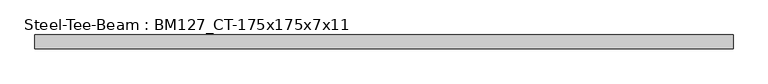
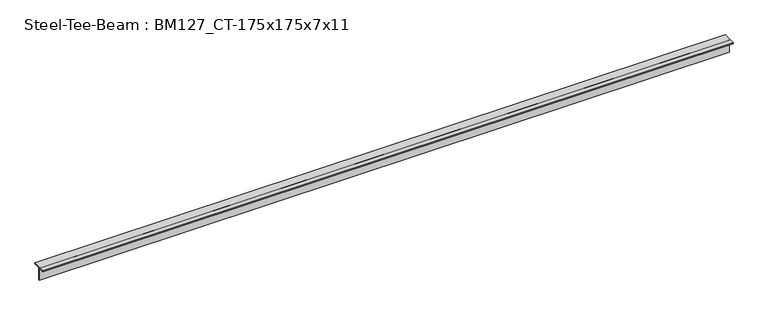
"""IFC4 building model written with IfcOpenShell, lengths in millimetres: beam geometry, Steel-Tee-Beam : BM127_CT-175x175x7x11."""

from ifc_helpers import new_model, si_unit, point, frame, frame_2d, origin, place, context, project, spatial, polyline, circle_curve, trimmed, segment, composite_curve, outline, extrude, source, transform, mapped, element, save


def steel_tee_beam_bm127_ct_175x175x7x11_3d5bc00e(model_context):
    return source(origin(), model_context, "Body", "SweptSolid", [
        extrude(outline(composite_curve([segment(polyline([(87.5, 87.5), (87.5, 76.5), (17.5, 76.5)]), True, "CONTINUOUS"), segment(trimmed(circle_curve(frame_2d((17.5, 62.5)), 14.0), [point((17.5, 76.5))], [point((3.5, 62.5))], True, "CARTESIAN"), True, "CONTINUOUS"), segment(polyline([(3.5, 62.5), (3.5, -87.5), (-3.5, -87.5), (-3.5, 62.5)]), True, "CONTINUOUS"), segment(trimmed(circle_curve(frame_2d((-17.5, 62.5)), 14.0), [point((-3.5, 62.5))], [point((-17.5, 76.5))], True, "CARTESIAN"), True, "CONTINUOUS"), segment(polyline([(-17.5, 76.5), (-87.5, 76.5), (-87.5, 87.5), (87.5, 87.5)]), True, "CONTINUOUS")], self_intersect=False)), frame((-4298.1792655, 0.0, 0.0), z_axis=(1.0, 0.0, 0.0), x_axis=(0.0, 1.0, 0.0)), (0.0, 0.0, 1.0), 8725.555017),
    ])


if __name__ == "__main__":
    model = new_model("IFC4")
    model_context = context("Model", 3, world=origin())
    ifc_project = project(units=[si_unit("LENGTHUNIT", "METRE", prefix="MILLI")], contexts=[model_context])
    site = spatial("IfcSite", under=ifc_project)
    building = spatial("IfcBuilding", under=site)
    placement = place(None, origin())
    steel_tee_beam_bm127_ct_175x175x7x11_shape = steel_tee_beam_bm127_ct_175x175x7x11_3d5bc00e(model_context)
    element("IfcBeam", 1, ObjectType="Steel-Tee-Beam : BM127_CT-175x175x7x11", at=placement, inside=building, context=model_context, shape_type="MappedRepresentation", body=[
        mapped(steel_tee_beam_bm127_ct_175x175x7x11_shape, transform((0.0, 0.0, 0.0), x_axis=(1.0, 0.0, 0.0), y_axis=(0.0, 1.0, 0.0), z_axis=(0.0, 0.0, 1.0))),
    ])
    save(model, "model.ifc")

# Revit data of these elements
# Type "Steel-Tee-Beam : BM127_CT-175x175x7x11"
#   Section Area = 31.57 cm²
#   Mass per Unit Length = 24.80 kg/m
#   Length [instance default] = 1524 mm
#   bf = 175 mm
#   d = 175 mm
#   k = 25 mm
#   kr = 14 mm
#   tf = 11 mm
#   tw = 7 mm
#   hec_material4 [instance default] = none
#   hec_material3 [instance default] = none
#   hec_material2 [instance default] = none
#   hec_material1 [instance default] = none
#   Structural Material [instance default] = Steel, 45-345
#   Assembly Code = ""
# Element 1 (IfcBeam, "Steel-Tee-Beam : BM127_CT-175x175x7x11")
#   hec_material3 = F01AC000-00002_Building/Shelter Fire Proofing Work_Intumescent Coating Type_1 hr. rating (UL 1709))
#   hec_material1 = S03AA029-00001_Main Steel Structure Erection Work_Shelter/Building_Light Steel
#   Structural Material = S01AA003-00001_Main Steel Structure Fabrication Work_Shelter/Building_Light Steel - Standard
#   Materials on its faces: "S01AA003-00001_Main Steel Structure Fabrication Work_Shelter/Building_Light Steel - Standard"
# Materials
#   "Steel, 45-345": class "Metal", colour RGB 189 187 185, transparency 0, Description = "Steel 345 MPa", Cost = 0
#   "S01AA003-00001_Main Steel Structure Fabrication Work_Shelter/Building_Light Steel - Standard": class "Metal", colour RGB 120 120 120, transparency 0, Comments = "(30KG/M>Weight)", Description = "Structural steel 50ksi", W00) Work Master Code = "S01AA003-00001", W01) Work Master_Lv1 = "Main Steel Structure Fabrication Work", W02) Work Master_Lv2 = "Shelter/Building", W03) Work Master_Spec.1 = "Light Steel - Standard (30KG/M>Weight)", Cost = 0
#   "F01AC000-00002_Building/Shelter Fire Proofing Work_Intumescent Coating Type_1 hr. rating (UL 1709))": class "Metal", colour RGB 255 128 128, transparency 0, Description = "Paint finished steel", W00) Work Master Code = "F01AC000-00002", W01) Work Master_Lv1 = "Building/Shelter Fire Proofing Work", W02) Work Master_Lv2 = "Intumescent Coating Type", W03) Work Master_Spec.1 = "1 hr. rating (UL 1709)", Cost = 0
#   "S03AA029-00001_Main Steel Structure Erection Work_Shelter/Building_Light Steel": class "Metal", colour RGB 120 120 120, transparency 0, Comments = "(30KG/M>Weight)", Description = "Structural steel 50ksi", W00) Work Master Code = "S03AA029-00001", W01) Work Master_Lv1 = "Main Steel Structure Erection Work", W02) Work Master_Lv2 = "Shelter/Building", W03) Work Master_Spec.1 = "Light Steel (30KG/M>Weight)", Cost = 0
